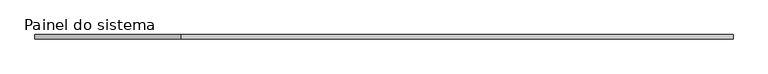
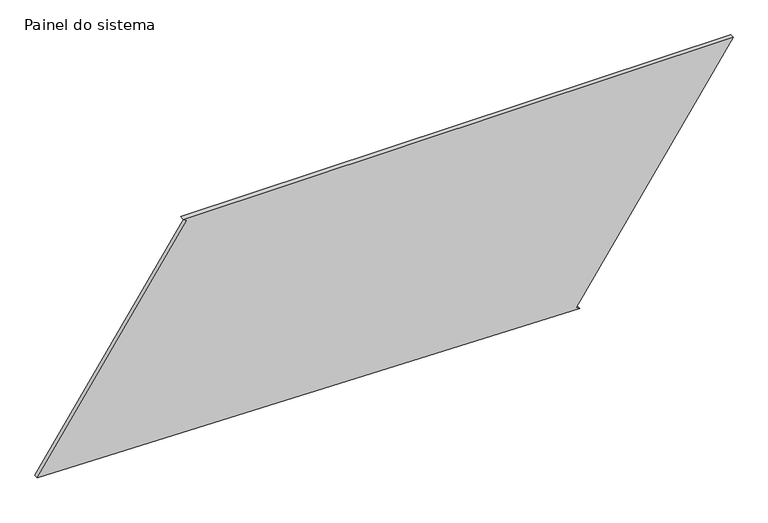
"""IFC4 building model written with IfcOpenShell, lengths in millimetres: plate geometry, Painel do sistema : Envidraçado."""

from ifc_helpers import new_model, si_unit, frame, origin, place, context, project, spatial, polyline, outline, extrude, source, transform, mapped, element, save


def painel_do_sistema_59143784(model_context):
    return source(origin(), model_context, "Body", "SweptSolid", [
        extrude(outline(polyline([(0.0, 1090.3415048), (14.052453, 1069.6647409), (1307.2941509, 1948.584587), (1307.2941509, -1131.7196502), (1293.2416979, -1111.0428863), (60.8837577, -1948.584587), (0.0, 1090.3415048)])), frame((0.0, 24.5, 0.0), z_axis=(0.0, 1.0, 0.0), x_axis=(0.0, 0.0, 1.0)), (0.0, 0.0, 1.0), 25.0),
    ])


if __name__ == "__main__":
    model = new_model("IFC4")
    model_context = context("Model", 3, world=origin())
    ifc_project = project(units=[si_unit("LENGTHUNIT", "METRE", prefix="MILLI")], contexts=[model_context])
    site = spatial("IfcSite", under=ifc_project)
    building = spatial("IfcBuilding", under=site)
    placement = place(None, origin())
    painel_do_sistema_shape = painel_do_sistema_59143784(model_context)
    element("IfcPlate", 1, ObjectType="Painel do sistema : Envidraçado", at=placement, inside=building, context=model_context, shape_type="MappedRepresentation", body=[
        mapped(painel_do_sistema_shape, transform((0.0, 0.0, 0.0), x_axis=(1.0, 0.0, 0.0), y_axis=(0.0, 1.0, 0.0), z_axis=(0.0, 0.0, 1.0))),
    ])
    save(model, "model.ifc")

# Revit data of these elements
# Type "Painel do sistema : Envidraçado"
#   Construction Type Id = "GSP4R"
#   Analytic Construction = "Vidraça única Pilkington 1/8 pol"
#   Visual Light Transmittance = 0.9
#   Solar Heat Gain Coefficient = 0.86
#   Heat Transfer Coefficient (U) = 6.7069 W/(m²·K)
# Element 1 (IfcPlate, "Painel do sistema : Envidraçado")
#   Materials on its faces: "Vidro"
# Materials
#   "Vidro": class "Vidro", colour RGB 0 128 192, transparency 0.9, Description = "Vidro de sílica", Cost = 0
